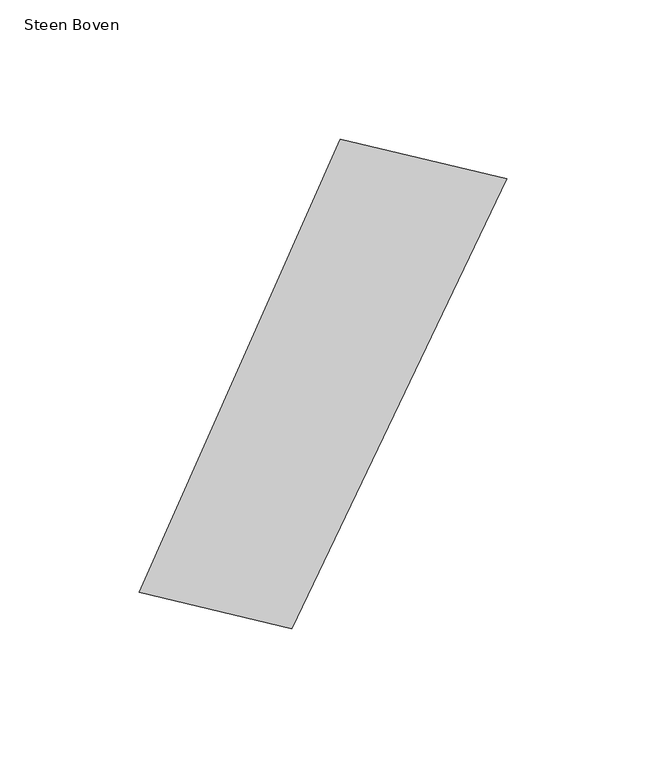
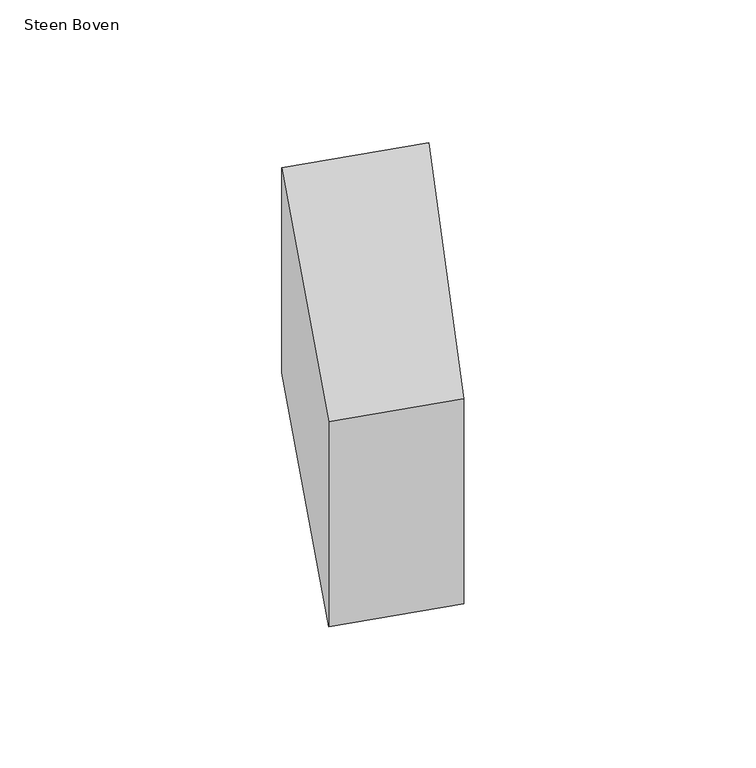
"""IFC4 building model written with IfcOpenShell, lengths in millimetres: proxy geometry, 00_GMA_steen_versie_4 : Steen Boven."""

from ifc_helpers import new_model, si_unit, origin, origin_with_axes, place, context, project, spatial, polyline, outline, extrude, source, transform, mapped, element, save


def steen_boven_d2a3f065(model_context):
    return source(origin(), model_context, "Body", "SweptSolid", [
        extrude(outline(polyline([(140.3455984, 152.8196075), (63.1886286, -8.7909873), (8.3154968, 4.3315664), (80.595855, 167.0827613), (140.3455984, 152.8196075)])), origin_with_axes(), (0.0, 0.0, 1.0), 100.0),
    ])


if __name__ == "__main__":
    model = new_model("IFC4")
    model_context = context("Model", 3, world=origin())
    ifc_project = project(units=[si_unit("LENGTHUNIT", "METRE", prefix="MILLI")], contexts=[model_context])
    site = spatial("IfcSite", under=ifc_project)
    building = spatial("IfcBuilding", under=site)
    placement = place(None, origin())
    steen_boven_shape = steen_boven_d2a3f065(model_context)
    element("IfcBuildingElementProxy", 1, Name="00_GMA_steen_versie_4 : Steen Boven", ObjectType="00_GMA_steen_versie_4 : Steen Boven", at=placement, inside=building, context=model_context, shape_type="MappedRepresentation", body=[
        mapped(steen_boven_shape, transform((0.0, 0.0, 0.0), x_axis=(1.0, 0.0, 0.0), y_axis=(0.0, 1.0, 0.0), z_axis=(0.0, 0.0, 1.0))),
    ])
    save(model, "model.ifc")

# Revit data of these elements
# Type "00_GMA_steen_versie_4 : Steen Boven"
#   StootVoegHalfBoven [instance default] = 5 mm
#   StootVoegHalf [instance default] = 5 mm
#   StootVoegBreedteOnder = 10 mm
#   StootVoegBreedteBoven = 10 mm
#   Steendikte = 100 mm
#   LintVoegOnderHalf = 5 mm
#   LintVoegOnder = 10 mm
#   LintVoegBovenHalf = 0 mm
#   LintVoegBoven = 0 mm
#   materiaal = none
#   MateriaalVoeg = none
#   Default Elevation = 0
